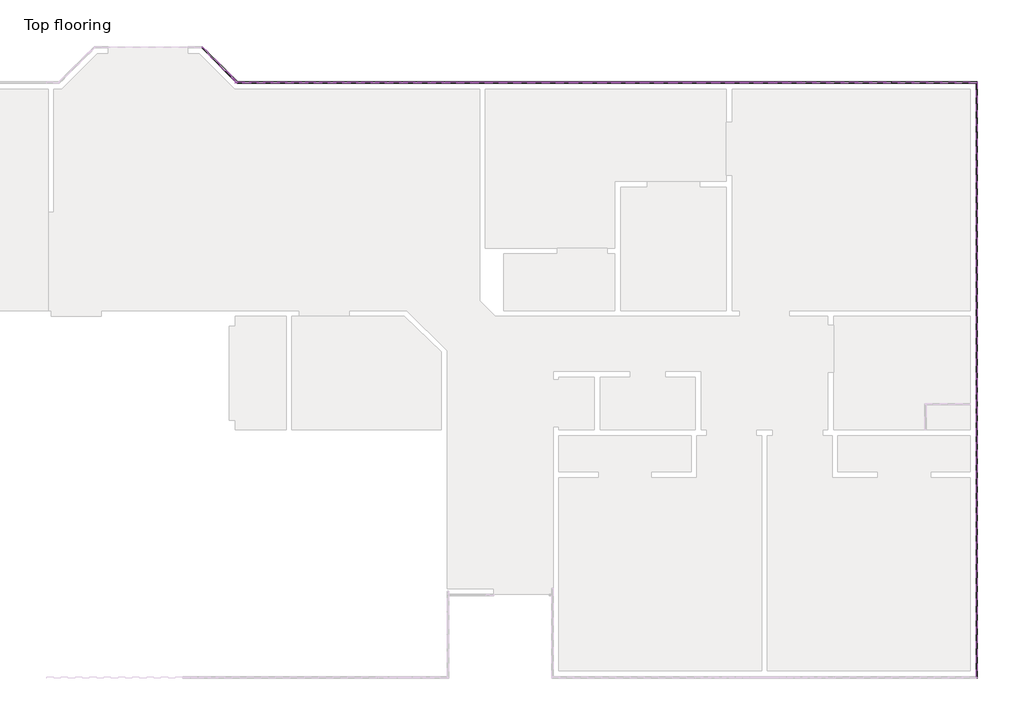
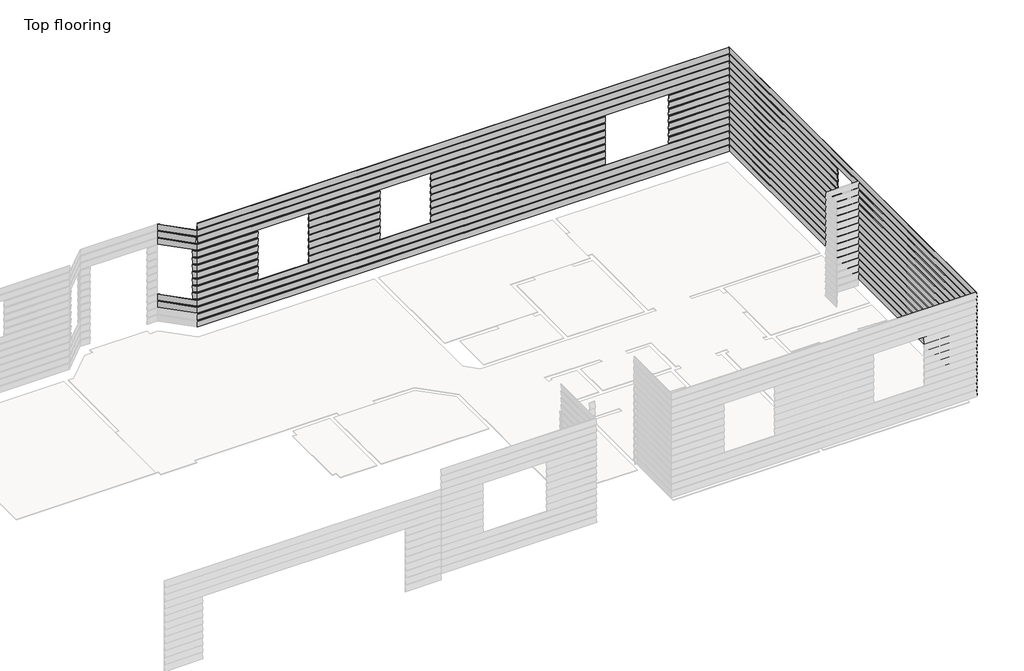
# One storey, part 5 of 5: 42 proxies.
"""IFC4 building model written with IfcOpenShell, lengths in millimetres."""

from ifc_helpers import new_model, si_unit, origin, place, context, project, spatial, faceted_brep, element, save

model = new_model("IFC4")

# Units and contexts
model_context = context("Model", 3, world=origin())
ifc_project = project(units=[si_unit("LENGTHUNIT", "METRE", prefix="MILLI")], contexts=[model_context])

# Site, building, storey
site = spatial("IfcSite", under=ifc_project)
building = spatial("IfcBuilding", under=site)
storey = spatial("IfcBuildingStorey", under=building, Name="Top flooring", Elevation=12.7)

# Proxies
placement = place(None, origin())
element("IfcBuildingElementProxy", 1, Name="Wall Sweeps", at=placement, inside=storey, context=model_context, shape_type="Brep", body=[
    faceted_brep([(-11064.5752841, 5231.8645018, 534.9151454), (-11070.4469329, 5217.6890875, 694.2859634), (-11074.5727801, 5207.7284114, 693.4), (-11068.7011312, 5221.9038257, 534.029182), (-11674.1752841, 5841.4645018, 534.9151454), (-11678.3011312, 5831.5038257, 534.029182), (-11684.1727801, 5817.3284114, 693.4), (-11680.0469329, 5827.2890875, 694.2859634)], [[[0, 1, 2, 3]], [[4, 5, 6, 7]], [[1, 0, 4, 7]], [[2, 1, 7, 6]], [[3, 2, 6, 5]], [[0, 3, 5, 4]]]),
])
element("IfcBuildingElementProxy", 2, Name="Wall Sweeps", at=placement, inside=storey, context=model_context, shape_type="Brep", body=[
    faceted_brep([(-11064.5752841, 5231.8645018, 712.7151454), (-11070.4469329, 5217.6890875, 872.0859634), (-11074.5727801, 5207.7284114, 871.2), (-11068.7011312, 5221.9038257, 711.829182), (-11674.1752841, 5841.4645018, 712.7151454), (-11678.3011312, 5831.5038257, 711.829182), (-11684.1727801, 5817.3284114, 871.2), (-11680.0469329, 5827.2890875, 872.0859634)], [[[0, 1, 2, 3]], [[4, 5, 6, 7]], [[1, 0, 4, 7]], [[2, 1, 7, 6]], [[3, 2, 6, 5]], [[0, 3, 5, 4]]]),
])
element("IfcBuildingElementProxy", 3, Name="Wall Sweeps", at=placement, inside=storey, context=model_context, shape_type="Brep", body=[
    faceted_brep([(-11064.5752841, 5231.8645018, 890.5151454), (-11070.4469329, 5217.6890875, 1049.8859634), (-11074.5727801, 5207.7284114, 1049.0), (-11068.7011312, 5221.9038257, 889.629182), (-11135.1593781, 5302.4485958, 890.5151454), (-11142.2026397, 5295.4053342, 889.629182), (-11152.2261713, 5285.3818026, 1049.0), (-11145.1829097, 5292.4250642, 1049.8859634)], [[[0, 1, 2, 3]], [[4, 5, 6, 7]], [[1, 0, 4, 7]], [[2, 1, 7, 6]], [[3, 2, 6, 5]], [[0, 3, 5, 4]]]),
])
element("IfcBuildingElementProxy", 4, Name="Wall Sweeps", at=placement, inside=storey, context=model_context, shape_type="Brep", body=[
    faceted_brep([(-11064.5752841, 5231.8645018, 1068.3151454), (-11070.4469329, 5217.6890875, 1227.6859634), (-11074.5727801, 5207.7284114, 1226.8), (-11068.7011312, 5221.9038257, 1067.429182), (-11135.1593781, 5302.4485958, 1068.3151454), (-11142.2026397, 5295.4053342, 1067.429182), (-11152.2261713, 5285.3818026, 1226.8), (-11145.1829097, 5292.4250642, 1227.6859634)], [[[0, 1, 2, 3]], [[4, 5, 6, 7]], [[1, 0, 4, 7]], [[2, 1, 7, 6]], [[3, 2, 6, 5]], [[0, 3, 5, 4]]]),
])
element("IfcBuildingElementProxy", 5, Name="Wall Sweeps", at=placement, inside=storey, context=model_context, shape_type="Brep", body=[
    faceted_brep([(-11064.5752841, 5231.8645018, 1246.1151454), (-11070.4469329, 5217.6890875, 1405.4859634), (-11074.5727801, 5207.7284114, 1404.6), (-11068.7011312, 5221.9038257, 1245.229182), (-11135.1593781, 5302.4485958, 1246.1151454), (-11142.2026397, 5295.4053342, 1245.229182), (-11152.2261713, 5285.3818026, 1404.6), (-11145.1829097, 5292.4250642, 1405.4859634)], [[[0, 1, 2, 3]], [[4, 5, 6, 7]], [[1, 0, 4, 7]], [[2, 1, 7, 6]], [[3, 2, 6, 5]], [[0, 3, 5, 4]]]),
])
element("IfcBuildingElementProxy", 6, Name="Wall Sweeps", at=placement, inside=storey, context=model_context, shape_type="Brep", body=[
    faceted_brep([(-11064.5752841, 5231.8645018, 1423.9151454), (-11070.4469329, 5217.6890875, 1583.2859634), (-11074.5727801, 5207.7284114, 1582.4), (-11068.7011312, 5221.9038257, 1423.029182), (-11135.1593781, 5302.4485958, 1423.9151454), (-11142.2026397, 5295.4053342, 1423.029182), (-11152.2261713, 5285.3818026, 1582.4), (-11145.1829097, 5292.4250642, 1583.2859634)], [[[0, 1, 2, 3]], [[4, 5, 6, 7]], [[1, 0, 4, 7]], [[2, 1, 7, 6]], [[3, 2, 6, 5]], [[0, 3, 5, 4]]]),
])
element("IfcBuildingElementProxy", 7, Name="Wall Sweeps", at=placement, inside=storey, context=model_context, shape_type="Brep", body=[
    faceted_brep([(-11064.5752841, 5231.8645018, 1601.7151454), (-11070.4469329, 5217.6890875, 1761.0859634), (-11074.5727801, 5207.7284114, 1760.2), (-11068.7011312, 5221.9038257, 1600.829182), (-11135.1593781, 5302.4485958, 1601.7151454), (-11142.2026397, 5295.4053342, 1600.829182), (-11152.2261713, 5285.3818026, 1760.2), (-11145.1829097, 5292.4250642, 1761.0859634)], [[[0, 1, 2, 3]], [[4, 5, 6, 7]], [[1, 0, 4, 7]], [[2, 1, 7, 6]], [[3, 2, 6, 5]], [[0, 3, 5, 4]]]),
])
element("IfcBuildingElementProxy", 8, Name="Wall Sweeps", at=placement, inside=storey, context=model_context, shape_type="Brep", body=[
    faceted_brep([(-11064.5752841, 5231.8645018, 1779.5151454), (-11070.4469329, 5217.6890875, 1938.8859634), (-11074.5727801, 5207.7284114, 1938.0), (-11068.7011312, 5221.9038257, 1778.629182), (-11135.1593781, 5302.4485958, 1779.5151454), (-11142.2026397, 5295.4053342, 1778.629182), (-11152.2261713, 5285.3818026, 1938.0), (-11145.1829097, 5292.4250642, 1938.8859634)], [[[0, 1, 2, 3]], [[4, 5, 6, 7]], [[1, 0, 4, 7]], [[2, 1, 7, 6]], [[3, 2, 6, 5]], [[0, 3, 5, 4]]]),
])
element("IfcBuildingElementProxy", 9, Name="Wall Sweeps", at=placement, inside=storey, context=model_context, shape_type="Brep", body=[
    faceted_brep([(-11064.5752841, 5231.8645018, 1957.3151454), (-11070.4469329, 5217.6890875, 2116.6859634), (-11074.5727801, 5207.7284114, 2115.8), (-11068.7011312, 5221.9038257, 1956.429182), (-11135.1593781, 5302.4485958, 1957.3151454), (-11142.2026397, 5295.4053342, 1956.429182), (-11152.2261713, 5285.3818026, 2115.8), (-11145.1829097, 5292.4250642, 2116.6859634)], [[[0, 1, 2, 3]], [[4, 5, 6, 7]], [[1, 0, 4, 7]], [[2, 1, 7, 6]], [[3, 2, 6, 5]], [[0, 3, 5, 4]]]),
])
element("IfcBuildingElementProxy", 10, Name="Wall Sweeps", at=placement, inside=storey, context=model_context, shape_type="Brep", body=[
    faceted_brep([(-11064.5752841, 5231.8645018, 2135.1151454), (-11070.4469329, 5217.6890875, 2294.4859634), (-11074.5727801, 5207.7284114, 2293.6), (-11068.7011312, 5221.9038257, 2134.229182), (-11674.1752841, 5841.4645018, 2135.1151454), (-11678.3011312, 5831.5038257, 2134.229182), (-11684.1727801, 5817.3284114, 2293.6), (-11680.0469329, 5827.2890875, 2294.4859634)], [[[0, 1, 2, 3]], [[4, 5, 6, 7]], [[1, 0, 4, 7]], [[2, 1, 7, 6]], [[3, 2, 6, 5]], [[0, 3, 5, 4]]]),
])
element("IfcBuildingElementProxy", 11, Name="Wall Sweeps", at=placement, inside=storey, context=model_context, shape_type="Brep", body=[
    faceted_brep([(1730.1212614, -5078.007679, 179.3151454), (1715.9458471, -5063.8322648, 338.6859634), (1705.985171, -5053.8715886, 337.8), (1720.1605853, -5068.0470029, 178.429182), (1730.1212614, 5231.8645018, 179.3151454), (1720.1605853, 5221.9038257, 178.429182), (1705.985171, 5207.7284114, 337.8), (1715.9458471, 5217.6890875, 338.6859634)], [[[0, 1, 2, 3]], [[4, 5, 6, 7]], [[1, 0, 4, 7]], [[2, 1, 7, 6]], [[3, 2, 6, 5]], [[0, 3, 5, 4]]]),
])
element("IfcBuildingElementProxy", 12, Name="Wall Sweeps", at=placement, inside=storey, context=model_context, shape_type="Brep", body=[
    faceted_brep([(1730.1212614, -5078.007679, 357.1151454), (1715.9458471, -5063.8322648, 516.4859634), (1705.985171, -5053.8715886, 515.6), (1720.1605853, -5068.0470029, 356.229182), (1730.1212614, 5231.8645018, 357.1151454), (1720.1605853, 5221.9038257, 356.229182), (1705.985171, 5207.7284114, 515.6), (1715.9458471, 5217.6890875, 516.4859634)], [[[0, 1, 2, 3]], [[4, 5, 6, 7]], [[1, 0, 4, 7]], [[2, 1, 7, 6]], [[3, 2, 6, 5]], [[0, 3, 5, 4]]]),
])
element("IfcBuildingElementProxy", 13, Name="Wall Sweeps", at=placement, inside=storey, context=model_context, shape_type="Brep", body=[
    faceted_brep([(1730.1212614, -5078.007679, 534.9151454), (1715.9458471, -5063.8322648, 694.2859634), (1705.985171, -5053.8715886, 693.4), (1720.1605853, -5068.0470029, 534.029182), (1730.1212614, 5231.8645018, 534.9151454), (1720.1605853, 5221.9038257, 534.029182), (1705.985171, 5207.7284114, 693.4), (1715.9458471, 5217.6890875, 694.2859634)], [[[0, 1, 2, 3]], [[4, 5, 6, 7]], [[1, 0, 4, 7]], [[2, 1, 7, 6]], [[3, 2, 6, 5]], [[0, 3, 5, 4]]]),
])
element("IfcBuildingElementProxy", 14, Name="Wall Sweeps", at=placement, inside=storey, context=model_context, shape_type="Brep", body=[
    faceted_brep([(1730.1212614, -5078.007679, 712.7151454), (1715.9458471, -5063.8322648, 872.0859634), (1705.985171, -5053.8715886, 871.2), (1720.1605853, -5068.0470029, 711.829182), (1730.1212614, 5231.8645018, 712.7151454), (1720.1605853, 5221.9038257, 711.829182), (1705.985171, 5207.7284114, 871.2), (1715.9458471, 5217.6890875, 872.0859634)], [[[0, 1, 2, 3]], [[4, 5, 6, 7]], [[1, 0, 4, 7]], [[2, 1, 7, 6]], [[3, 2, 6, 5]], [[0, 3, 5, 4]]]),
])
element("IfcBuildingElementProxy", 15, Name="Wall Sweeps", at=placement, inside=storey, context=model_context, shape_type="Brep", body=[
    faceted_brep([(1730.1212614, -5078.007679, 890.5151454), (1715.9458471, -5063.8322648, 1049.8859634), (1705.985171, -5053.8715886, 1049.0), (1720.1605853, -5068.0470029, 889.629182), (1730.1212614, 5231.8645018, 890.5151454), (1720.1605853, 5221.9038257, 889.629182), (1705.985171, 5207.7284114, 1049.0), (1715.9458471, 5217.6890875, 1049.8859634)], [[[0, 1, 2, 3]], [[4, 5, 6, 7]], [[1, 0, 4, 7]], [[2, 1, 7, 6]], [[3, 2, 6, 5]], [[0, 3, 5, 4]]]),
])
element("IfcBuildingElementProxy", 16, Name="Wall Sweeps", at=placement, inside=storey, context=model_context, shape_type="Brep", body=[
    faceted_brep([(1730.1212614, -5078.007679, 1068.3151454), (1715.9458471, -5063.8322648, 1227.6859634), (1705.985171, -5053.8715886, 1226.8), (1720.1605853, -5068.0470029, 1067.429182), (1730.1212614, 5231.8645018, 1068.3151454), (1720.1605853, 5221.9038257, 1067.429182), (1705.985171, 5207.7284114, 1226.8), (1715.9458471, 5217.6890875, 1227.6859634)], [[[0, 1, 2, 3]], [[4, 5, 6, 7]], [[1, 0, 4, 7]], [[2, 1, 7, 6]], [[3, 2, 6, 5]], [[0, 3, 5, 4]]]),
])
element("IfcBuildingElementProxy", 17, Name="Wall Sweeps", at=placement, inside=storey, context=model_context, shape_type="Brep", body=[
    faceted_brep([(1730.1212614, -5078.007679, 1246.1151454), (1715.9458471, -5063.8322648, 1405.4859634), (1705.985171, -5053.8715886, 1404.6), (1720.1605853, -5068.0470029, 1245.229182), (1730.1212614, 5231.8645018, 1246.1151454), (1720.1605853, 5221.9038257, 1245.229182), (1705.985171, 5207.7284114, 1404.6), (1715.9458471, 5217.6890875, 1405.4859634)], [[[0, 1, 2, 3]], [[4, 5, 6, 7]], [[1, 0, 4, 7]], [[2, 1, 7, 6]], [[3, 2, 6, 5]], [[0, 3, 5, 4]]]),
])
element("IfcBuildingElementProxy", 18, Name="Wall Sweeps", at=placement, inside=storey, context=model_context, shape_type="Brep", body=[
    faceted_brep([(1730.1212614, -5078.007679, 1423.9151454), (1715.9458471, -5063.8322648, 1583.2859634), (1705.985171, -5053.8715886, 1582.4), (1720.1605853, -5068.0470029, 1423.029182), (1730.1212614, 5231.8645018, 1423.9151454), (1720.1605853, 5221.9038257, 1423.029182), (1705.985171, 5207.7284114, 1582.4), (1715.9458471, 5217.6890875, 1583.2859634)], [[[0, 1, 2, 3]], [[4, 5, 6, 7]], [[1, 0, 4, 7]], [[2, 1, 7, 6]], [[3, 2, 6, 5]], [[0, 3, 5, 4]]]),
])
element("IfcBuildingElementProxy", 19, Name="Wall Sweeps", at=placement, inside=storey, context=model_context, shape_type="Brep", body=[
    faceted_brep([(1730.1212614, -5078.007679, 1601.7151454), (1715.9458471, -5063.8322648, 1761.0859634), (1705.985171, -5053.8715886, 1760.2), (1720.1605853, -5068.0470029, 1600.829182), (1730.1212614, 5231.8645018, 1601.7151454), (1720.1605853, 5221.9038257, 1600.829182), (1705.985171, 5207.7284114, 1760.2), (1715.9458471, 5217.6890875, 1761.0859634)], [[[0, 1, 2, 3]], [[4, 5, 6, 7]], [[1, 0, 4, 7]], [[2, 1, 7, 6]], [[3, 2, 6, 5]], [[0, 3, 5, 4]]]),
])
element("IfcBuildingElementProxy", 20, Name="Wall Sweeps", at=placement, inside=storey, context=model_context, shape_type="Brep", body=[
    faceted_brep([(1730.1212614, -5078.007679, 1779.5151454), (1715.9458471, -5063.8322648, 1938.8859634), (1705.985171, -5053.8715886, 1938.0), (1720.1605853, -5068.0470029, 1778.629182), (1730.1212614, 5231.8645018, 1779.5151454), (1720.1605853, 5221.9038257, 1778.629182), (1705.985171, 5207.7284114, 1938.0), (1715.9458471, 5217.6890875, 1938.8859634)], [[[0, 1, 2, 3]], [[4, 5, 6, 7]], [[1, 0, 4, 7]], [[2, 1, 7, 6]], [[3, 2, 6, 5]], [[0, 3, 5, 4]]]),
])
element("IfcBuildingElementProxy", 21, Name="Wall Sweeps", at=placement, inside=storey, context=model_context, shape_type="Brep", body=[
    faceted_brep([(1730.1212614, -5078.007679, 1957.3151454), (1715.9458471, -5063.8322648, 2116.6859634), (1705.985171, -5053.8715886, 2115.8), (1720.1605853, -5068.0470029, 1956.429182), (1730.1212614, 102.3284114, 1957.3151454), (1720.1605853, 102.3284114, 1956.429182), (1705.985171, 102.3284114, 2115.8), (1715.9458471, 102.3284114, 2116.6859634)], [[[0, 1, 2, 3]], [[4, 5, 6, 7]], [[1, 0, 4, 7]], [[2, 1, 7, 6]], [[3, 2, 6, 5]], [[0, 3, 5, 4]]]),
    faceted_brep([(1730.1212614, 711.9284114, 1957.3151454), (1715.9458471, 711.9284114, 2116.6859634), (1705.985171, 711.9284114, 2115.8), (1720.1605853, 711.9284114, 1956.429182), (1730.1212614, 5231.8645018, 1957.3151454), (1720.1605853, 5221.9038257, 1956.429182), (1705.985171, 5207.7284114, 2115.8), (1715.9458471, 5217.6890875, 2116.6859634)], [[[0, 1, 2, 3]], [[4, 5, 6, 7]], [[1, 0, 4, 7]], [[2, 1, 7, 6]], [[3, 2, 6, 5]], [[0, 3, 5, 4]]]),
])
element("IfcBuildingElementProxy", 22, Name="Wall Sweeps", at=placement, inside=storey, context=model_context, shape_type="Brep", body=[
    faceted_brep([(1730.1212614, -5078.007679, 2135.1151454), (1715.9458471, -5063.8322648, 2294.4859634), (1705.985171, -5053.8715886, 2293.6), (1720.1605853, -5068.0470029, 2134.229182), (1730.1212614, 102.3284114, 2135.1151454), (1720.1605853, 102.3284114, 2134.229182), (1705.985171, 102.3284114, 2293.6), (1715.9458471, 102.3284114, 2294.4859634)], [[[0, 1, 2, 3]], [[4, 5, 6, 7]], [[1, 0, 4, 7]], [[2, 1, 7, 6]], [[3, 2, 6, 5]], [[0, 3, 5, 4]]]),
    faceted_brep([(1730.1212614, 711.9284114, 2135.1151454), (1715.9458471, 711.9284114, 2294.4859634), (1705.985171, 711.9284114, 2293.6), (1720.1605853, 711.9284114, 2134.229182), (1730.1212614, 5231.8645018, 2135.1151454), (1720.1605853, 5221.9038257, 2134.229182), (1705.985171, 5207.7284114, 2293.6), (1715.9458471, 5217.6890875, 2294.4859634)], [[[0, 1, 2, 3]], [[4, 5, 6, 7]], [[1, 0, 4, 7]], [[2, 1, 7, 6]], [[3, 2, 6, 5]], [[0, 3, 5, 4]]]),
])
element("IfcBuildingElementProxy", 23, Name="Wall Sweeps", at=placement, inside=storey, context=model_context, shape_type="Brep", body=[
    faceted_brep([(1730.1212614, 5231.8645018, 179.3151454), (1715.9458471, 5217.6890875, 338.6859634), (1705.985171, 5207.7284114, 337.8), (1720.1605853, 5221.9038257, 178.429182), (-11064.5752841, 5231.8645018, 179.3151454), (-11068.7011312, 5221.9038257, 178.429182), (-11074.5727801, 5207.7284114, 337.8), (-11070.4469329, 5217.6890875, 338.6859634)], [[[0, 1, 2, 3]], [[4, 5, 6, 7]], [[1, 0, 4, 7]], [[2, 1, 7, 6]], [[3, 2, 6, 5]], [[0, 3, 5, 4]]]),
])
element("IfcBuildingElementProxy", 24, Name="Wall Sweeps", at=placement, inside=storey, context=model_context, shape_type="Brep", body=[
    faceted_brep([(1730.1212614, 5231.8645018, 357.1151454), (1715.9458471, 5217.6890875, 516.4859634), (1705.985171, 5207.7284114, 515.6), (1720.1605853, 5221.9038257, 356.229182), (-11064.5752841, 5231.8645018, 357.1151454), (-11068.7011312, 5221.9038257, 356.229182), (-11074.5727801, 5207.7284114, 515.6), (-11070.4469329, 5217.6890875, 516.4859634)], [[[0, 1, 2, 3]], [[4, 5, 6, 7]], [[1, 0, 4, 7]], [[2, 1, 7, 6]], [[3, 2, 6, 5]], [[0, 3, 5, 4]]]),
])
element("IfcBuildingElementProxy", 25, Name="Wall Sweeps", at=placement, inside=storey, context=model_context, shape_type="Brep", body=[
    faceted_brep([(1730.1212614, 5231.8645018, 534.9151454), (1715.9458471, 5217.6890875, 694.2859634), (1705.985171, 5207.7284114, 693.4), (1720.1605853, 5221.9038257, 534.029182), (-11064.5752841, 5231.8645018, 534.9151454), (-11068.7011312, 5221.9038257, 534.029182), (-11074.5727801, 5207.7284114, 693.4), (-11070.4469329, 5217.6890875, 694.2859634)], [[[0, 1, 2, 3]], [[4, 5, 6, 7]], [[1, 0, 4, 7]], [[2, 1, 7, 6]], [[3, 2, 6, 5]], [[0, 3, 5, 4]]]),
])
element("IfcBuildingElementProxy", 26, Name="Wall Sweeps", at=placement, inside=storey, context=model_context, shape_type="Brep", body=[
    faceted_brep([(1730.1212614, 5231.8645018, 712.7151454), (1715.9458471, 5217.6890875, 872.0859634), (1705.985171, 5207.7284114, 871.2), (1720.1605853, 5221.9038257, 711.829182), (-11064.5752841, 5231.8645018, 712.7151454), (-11068.7011312, 5221.9038257, 711.829182), (-11074.5727801, 5207.7284114, 871.2), (-11070.4469329, 5217.6890875, 872.0859634)], [[[0, 1, 2, 3]], [[4, 5, 6, 7]], [[1, 0, 4, 7]], [[2, 1, 7, 6]], [[3, 2, 6, 5]], [[0, 3, 5, 4]]]),
])
element("IfcBuildingElementProxy", 27, Name="Wall Sweeps", at=placement, inside=storey, context=model_context, shape_type="Brep", body=[
    faceted_brep([(1730.1212614, 5231.8645018, 890.5151454), (1715.9458471, 5217.6890875, 1049.8859634), (1705.985171, 5207.7284114, 1049.0), (1720.1605853, 5221.9038257, 889.629182), (251.835171, 5231.8645018, 890.5151454), (251.835171, 5221.9038257, 889.629182), (251.835171, 5207.7284114, 1049.0), (251.835171, 5217.6890875, 1049.8859634)], [[[0, 1, 2, 3]], [[4, 5, 6, 7]], [[1, 0, 4, 7]], [[2, 1, 7, 6]], [[3, 2, 6, 5]], [[0, 3, 5, 4]]]),
    faceted_brep([(-1272.164829, 5231.8645018, 890.5151454), (-1272.164829, 5217.6890875, 1049.8859634), (-1272.164829, 5207.7284114, 1049.0), (-1272.164829, 5221.9038257, 889.629182), (-5463.164829, 5231.8645018, 890.5151454), (-5463.164829, 5221.9038257, 889.629182), (-5463.164829, 5207.7284114, 1049.0), (-5463.164829, 5217.6890875, 1049.8859634)], [[[0, 1, 2, 3]], [[4, 5, 6, 7]], [[1, 0, 4, 7]], [[2, 1, 7, 6]], [[3, 2, 6, 5]], [[0, 3, 5, 4]]]),
    faceted_brep([(-6682.364829, 5231.8645018, 890.5151454), (-6682.364829, 5217.6890875, 1049.8859634), (-6682.364829, 5207.7284114, 1049.0), (-6682.364829, 5221.9038257, 889.629182), (-8396.864829, 5231.8645018, 890.5151454), (-8396.864829, 5221.9038257, 889.629182), (-8396.864829, 5207.7284114, 1049.0), (-8396.864829, 5217.6890875, 1049.8859634)], [[[0, 1, 2, 3]], [[4, 5, 6, 7]], [[1, 0, 4, 7]], [[2, 1, 7, 6]], [[3, 2, 6, 5]], [[0, 3, 5, 4]]]),
    faceted_brep([(-9616.064829, 5231.8645018, 890.5151454), (-9616.064829, 5217.6890875, 1049.8859634), (-9616.064829, 5207.7284114, 1049.0), (-9616.064829, 5221.9038257, 889.629182), (-11064.5752841, 5231.8645018, 890.5151454), (-11068.7011312, 5221.9038257, 889.629182), (-11074.5727801, 5207.7284114, 1049.0), (-11070.4469329, 5217.6890875, 1049.8859634)], [[[0, 1, 2, 3]], [[4, 5, 6, 7]], [[1, 0, 4, 7]], [[2, 1, 7, 6]], [[3, 2, 6, 5]], [[0, 3, 5, 4]]]),
])
element("IfcBuildingElementProxy", 28, Name="Wall Sweeps", at=placement, inside=storey, context=model_context, shape_type="Brep", body=[
    faceted_brep([(-9616.064829, 5231.8645018, 1068.3151454), (-9616.064829, 5217.6890875, 1227.6859634), (-9616.064829, 5207.7284114, 1226.8), (-9616.064829, 5221.9038257, 1067.429182), (-11064.5752841, 5231.8645018, 1068.3151454), (-11068.7011312, 5221.9038257, 1067.429182), (-11074.5727801, 5207.7284114, 1226.8), (-11070.4469329, 5217.6890875, 1227.6859634)], [[[0, 1, 2, 3]], [[4, 5, 6, 7]], [[1, 0, 4, 7]], [[2, 1, 7, 6]], [[3, 2, 6, 5]], [[0, 3, 5, 4]]]),
    faceted_brep([(-6682.364829, 5231.8645018, 1068.3151454), (-6682.364829, 5217.6890875, 1227.6859634), (-6682.364829, 5207.7284114, 1226.8), (-6682.364829, 5221.9038257, 1067.429182), (-8396.864829, 5231.8645018, 1068.3151454), (-8396.864829, 5221.9038257, 1067.429182), (-8396.864829, 5207.7284114, 1226.8), (-8396.864829, 5217.6890875, 1227.6859634)], [[[0, 1, 2, 3]], [[4, 5, 6, 7]], [[1, 0, 4, 7]], [[2, 1, 7, 6]], [[3, 2, 6, 5]], [[0, 3, 5, 4]]]),
    faceted_brep([(-1272.164829, 5231.8645018, 1068.3151454), (-1272.164829, 5217.6890875, 1227.6859634), (-1272.164829, 5207.7284114, 1226.8), (-1272.164829, 5221.9038257, 1067.429182), (-5463.164829, 5231.8645018, 1068.3151454), (-5463.164829, 5221.9038257, 1067.429182), (-5463.164829, 5207.7284114, 1226.8), (-5463.164829, 5217.6890875, 1227.6859634)], [[[0, 1, 2, 3]], [[4, 5, 6, 7]], [[1, 0, 4, 7]], [[2, 1, 7, 6]], [[3, 2, 6, 5]], [[0, 3, 5, 4]]]),
    faceted_brep([(1730.1212614, 5231.8645018, 1068.3151454), (1715.9458471, 5217.6890875, 1227.6859634), (1705.985171, 5207.7284114, 1226.8), (1720.1605853, 5221.9038257, 1067.429182), (251.835171, 5231.8645018, 1068.3151454), (251.835171, 5221.9038257, 1067.429182), (251.835171, 5207.7284114, 1226.8), (251.835171, 5217.6890875, 1227.6859634)], [[[0, 1, 2, 3]], [[4, 5, 6, 7]], [[1, 0, 4, 7]], [[2, 1, 7, 6]], [[3, 2, 6, 5]], [[0, 3, 5, 4]]]),
])
element("IfcBuildingElementProxy", 29, Name="Wall Sweeps", at=placement, inside=storey, context=model_context, shape_type="Brep", body=[
    faceted_brep([(-9616.064829, 5231.8645018, 1246.1151454), (-9616.064829, 5217.6890875, 1405.4859634), (-9616.064829, 5207.7284114, 1404.6), (-9616.064829, 5221.9038257, 1245.229182), (-11064.5752841, 5231.8645018, 1246.1151454), (-11068.7011312, 5221.9038257, 1245.229182), (-11074.5727801, 5207.7284114, 1404.6), (-11070.4469329, 5217.6890875, 1405.4859634)], [[[0, 1, 2, 3]], [[4, 5, 6, 7]], [[1, 0, 4, 7]], [[2, 1, 7, 6]], [[3, 2, 6, 5]], [[0, 3, 5, 4]]]),
    faceted_brep([(-6682.364829, 5231.8645018, 1246.1151454), (-6682.364829, 5217.6890875, 1405.4859634), (-6682.364829, 5207.7284114, 1404.6), (-6682.364829, 5221.9038257, 1245.229182), (-8396.864829, 5231.8645018, 1246.1151454), (-8396.864829, 5221.9038257, 1245.229182), (-8396.864829, 5207.7284114, 1404.6), (-8396.864829, 5217.6890875, 1405.4859634)], [[[0, 1, 2, 3]], [[4, 5, 6, 7]], [[1, 0, 4, 7]], [[2, 1, 7, 6]], [[3, 2, 6, 5]], [[0, 3, 5, 4]]]),
    faceted_brep([(-1272.164829, 5231.8645018, 1246.1151454), (-1272.164829, 5217.6890875, 1405.4859634), (-1272.164829, 5207.7284114, 1404.6), (-1272.164829, 5221.9038257, 1245.229182), (-5463.164829, 5231.8645018, 1246.1151454), (-5463.164829, 5221.9038257, 1245.229182), (-5463.164829, 5207.7284114, 1404.6), (-5463.164829, 5217.6890875, 1405.4859634)], [[[0, 1, 2, 3]], [[4, 5, 6, 7]], [[1, 0, 4, 7]], [[2, 1, 7, 6]], [[3, 2, 6, 5]], [[0, 3, 5, 4]]]),
    faceted_brep([(1730.1212614, 5231.8645018, 1246.1151454), (1715.9458471, 5217.6890875, 1405.4859634), (1705.985171, 5207.7284114, 1404.6), (1720.1605853, 5221.9038257, 1245.229182), (251.835171, 5231.8645018, 1246.1151454), (251.835171, 5221.9038257, 1245.229182), (251.835171, 5207.7284114, 1404.6), (251.835171, 5217.6890875, 1405.4859634)], [[[0, 1, 2, 3]], [[4, 5, 6, 7]], [[1, 0, 4, 7]], [[2, 1, 7, 6]], [[3, 2, 6, 5]], [[0, 3, 5, 4]]]),
])
element("IfcBuildingElementProxy", 30, Name="Wall Sweeps", at=placement, inside=storey, context=model_context, shape_type="Brep", body=[
    faceted_brep([(-9616.064829, 5231.8645018, 1423.9151454), (-9616.064829, 5217.6890875, 1583.2859634), (-9616.064829, 5207.7284114, 1582.4), (-9616.064829, 5221.9038257, 1423.029182), (-11064.5752841, 5231.8645018, 1423.9151454), (-11068.7011312, 5221.9038257, 1423.029182), (-11074.5727801, 5207.7284114, 1582.4), (-11070.4469329, 5217.6890875, 1583.2859634)], [[[0, 1, 2, 3]], [[4, 5, 6, 7]], [[1, 0, 4, 7]], [[2, 1, 7, 6]], [[3, 2, 6, 5]], [[0, 3, 5, 4]]]),
    faceted_brep([(-6682.364829, 5231.8645018, 1423.9151454), (-6682.364829, 5217.6890875, 1583.2859634), (-6682.364829, 5207.7284114, 1582.4), (-6682.364829, 5221.9038257, 1423.029182), (-8396.864829, 5231.8645018, 1423.9151454), (-8396.864829, 5221.9038257, 1423.029182), (-8396.864829, 5207.7284114, 1582.4), (-8396.864829, 5217.6890875, 1583.2859634)], [[[0, 1, 2, 3]], [[4, 5, 6, 7]], [[1, 0, 4, 7]], [[2, 1, 7, 6]], [[3, 2, 6, 5]], [[0, 3, 5, 4]]]),
    faceted_brep([(-1272.164829, 5231.8645018, 1423.9151454), (-1272.164829, 5217.6890875, 1583.2859634), (-1272.164829, 5207.7284114, 1582.4), (-1272.164829, 5221.9038257, 1423.029182), (-5463.164829, 5231.8645018, 1423.9151454), (-5463.164829, 5221.9038257, 1423.029182), (-5463.164829, 5207.7284114, 1582.4), (-5463.164829, 5217.6890875, 1583.2859634)], [[[0, 1, 2, 3]], [[4, 5, 6, 7]], [[1, 0, 4, 7]], [[2, 1, 7, 6]], [[3, 2, 6, 5]], [[0, 3, 5, 4]]]),
    faceted_brep([(1730.1212614, 5231.8645018, 1423.9151454), (1715.9458471, 5217.6890875, 1583.2859634), (1705.985171, 5207.7284114, 1582.4), (1720.1605853, 5221.9038257, 1423.029182), (251.835171, 5231.8645018, 1423.9151454), (251.835171, 5221.9038257, 1423.029182), (251.835171, 5207.7284114, 1582.4), (251.835171, 5217.6890875, 1583.2859634)], [[[0, 1, 2, 3]], [[4, 5, 6, 7]], [[1, 0, 4, 7]], [[2, 1, 7, 6]], [[3, 2, 6, 5]], [[0, 3, 5, 4]]]),
])
element("IfcBuildingElementProxy", 31, Name="Wall Sweeps", at=placement, inside=storey, context=model_context, shape_type="Brep", body=[
    faceted_brep([(-9616.064829, 5231.8645018, 1601.7151454), (-9616.064829, 5217.6890875, 1761.0859634), (-9616.064829, 5207.7284114, 1760.2), (-9616.064829, 5221.9038257, 1600.829182), (-11064.5752841, 5231.8645018, 1601.7151454), (-11068.7011312, 5221.9038257, 1600.829182), (-11074.5727801, 5207.7284114, 1760.2), (-11070.4469329, 5217.6890875, 1761.0859634)], [[[0, 1, 2, 3]], [[4, 5, 6, 7]], [[1, 0, 4, 7]], [[2, 1, 7, 6]], [[3, 2, 6, 5]], [[0, 3, 5, 4]]]),
    faceted_brep([(-6682.364829, 5231.8645018, 1601.7151454), (-6682.364829, 5217.6890875, 1761.0859634), (-6682.364829, 5207.7284114, 1760.2), (-6682.364829, 5221.9038257, 1600.829182), (-8396.864829, 5231.8645018, 1601.7151454), (-8396.864829, 5221.9038257, 1600.829182), (-8396.864829, 5207.7284114, 1760.2), (-8396.864829, 5217.6890875, 1761.0859634)], [[[0, 1, 2, 3]], [[4, 5, 6, 7]], [[1, 0, 4, 7]], [[2, 1, 7, 6]], [[3, 2, 6, 5]], [[0, 3, 5, 4]]]),
    faceted_brep([(-1272.164829, 5231.8645018, 1601.7151454), (-1272.164829, 5217.6890875, 1761.0859634), (-1272.164829, 5207.7284114, 1760.2), (-1272.164829, 5221.9038257, 1600.829182), (-5463.164829, 5231.8645018, 1601.7151454), (-5463.164829, 5221.9038257, 1600.829182), (-5463.164829, 5207.7284114, 1760.2), (-5463.164829, 5217.6890875, 1761.0859634)], [[[0, 1, 2, 3]], [[4, 5, 6, 7]], [[1, 0, 4, 7]], [[2, 1, 7, 6]], [[3, 2, 6, 5]], [[0, 3, 5, 4]]]),
    faceted_brep([(1730.1212614, 5231.8645018, 1601.7151454), (1715.9458471, 5217.6890875, 1761.0859634), (1705.985171, 5207.7284114, 1760.2), (1720.1605853, 5221.9038257, 1600.829182), (251.835171, 5231.8645018, 1601.7151454), (251.835171, 5221.9038257, 1600.829182), (251.835171, 5207.7284114, 1760.2), (251.835171, 5217.6890875, 1761.0859634)], [[[0, 1, 2, 3]], [[4, 5, 6, 7]], [[1, 0, 4, 7]], [[2, 1, 7, 6]], [[3, 2, 6, 5]], [[0, 3, 5, 4]]]),
])
element("IfcBuildingElementProxy", 32, Name="Wall Sweeps", at=placement, inside=storey, context=model_context, shape_type="Brep", body=[
    faceted_brep([(-9616.064829, 5231.8645018, 1779.5151454), (-9616.064829, 5217.6890875, 1938.8859634), (-9616.064829, 5207.7284114, 1938.0), (-9616.064829, 5221.9038257, 1778.629182), (-11064.5752841, 5231.8645018, 1779.5151454), (-11068.7011312, 5221.9038257, 1778.629182), (-11074.5727801, 5207.7284114, 1938.0), (-11070.4469329, 5217.6890875, 1938.8859634)], [[[0, 1, 2, 3]], [[4, 5, 6, 7]], [[1, 0, 4, 7]], [[2, 1, 7, 6]], [[3, 2, 6, 5]], [[0, 3, 5, 4]]]),
    faceted_brep([(-6682.364829, 5231.8645018, 1779.5151454), (-6682.364829, 5217.6890875, 1938.8859634), (-6682.364829, 5207.7284114, 1938.0), (-6682.364829, 5221.9038257, 1778.629182), (-8396.864829, 5231.8645018, 1779.5151454), (-8396.864829, 5221.9038257, 1778.629182), (-8396.864829, 5207.7284114, 1938.0), (-8396.864829, 5217.6890875, 1938.8859634)], [[[0, 1, 2, 3]], [[4, 5, 6, 7]], [[1, 0, 4, 7]], [[2, 1, 7, 6]], [[3, 2, 6, 5]], [[0, 3, 5, 4]]]),
    faceted_brep([(-1272.164829, 5231.8645018, 1779.5151454), (-1272.164829, 5217.6890875, 1938.8859634), (-1272.164829, 5207.7284114, 1938.0), (-1272.164829, 5221.9038257, 1778.629182), (-5463.164829, 5231.8645018, 1779.5151454), (-5463.164829, 5221.9038257, 1778.629182), (-5463.164829, 5207.7284114, 1938.0), (-5463.164829, 5217.6890875, 1938.8859634)], [[[0, 1, 2, 3]], [[4, 5, 6, 7]], [[1, 0, 4, 7]], [[2, 1, 7, 6]], [[3, 2, 6, 5]], [[0, 3, 5, 4]]]),
    faceted_brep([(1730.1212614, 5231.8645018, 1779.5151454), (1715.9458471, 5217.6890875, 1938.8859634), (1705.985171, 5207.7284114, 1938.0), (1720.1605853, 5221.9038257, 1778.629182), (251.835171, 5231.8645018, 1779.5151454), (251.835171, 5221.9038257, 1778.629182), (251.835171, 5207.7284114, 1938.0), (251.835171, 5217.6890875, 1938.8859634)], [[[0, 1, 2, 3]], [[4, 5, 6, 7]], [[1, 0, 4, 7]], [[2, 1, 7, 6]], [[3, 2, 6, 5]], [[0, 3, 5, 4]]]),
])
element("IfcBuildingElementProxy", 33, Name="Wall Sweeps", at=placement, inside=storey, context=model_context, shape_type="Brep", body=[
    faceted_brep([(-9616.064829, 5231.8645018, 1957.3151454), (-9616.064829, 5217.6890875, 2116.6859634), (-9616.064829, 5207.7284114, 2115.8), (-9616.064829, 5221.9038257, 1956.429182), (-11064.5752841, 5231.8645018, 1957.3151454), (-11068.7011312, 5221.9038257, 1956.429182), (-11074.5727801, 5207.7284114, 2115.8), (-11070.4469329, 5217.6890875, 2116.6859634)], [[[0, 1, 2, 3]], [[4, 5, 6, 7]], [[1, 0, 4, 7]], [[2, 1, 7, 6]], [[3, 2, 6, 5]], [[0, 3, 5, 4]]]),
    faceted_brep([(-6682.364829, 5231.8645018, 1957.3151454), (-6682.364829, 5217.6890875, 2116.6859634), (-6682.364829, 5207.7284114, 2115.8), (-6682.364829, 5221.9038257, 1956.429182), (-8396.864829, 5231.8645018, 1957.3151454), (-8396.864829, 5221.9038257, 1956.429182), (-8396.864829, 5207.7284114, 2115.8), (-8396.864829, 5217.6890875, 2116.6859634)], [[[0, 1, 2, 3]], [[4, 5, 6, 7]], [[1, 0, 4, 7]], [[2, 1, 7, 6]], [[3, 2, 6, 5]], [[0, 3, 5, 4]]]),
    faceted_brep([(-1272.164829, 5231.8645018, 1957.3151454), (-1272.164829, 5217.6890875, 2116.6859634), (-1272.164829, 5207.7284114, 2115.8), (-1272.164829, 5221.9038257, 1956.429182), (-5463.164829, 5231.8645018, 1957.3151454), (-5463.164829, 5221.9038257, 1956.429182), (-5463.164829, 5207.7284114, 2115.8), (-5463.164829, 5217.6890875, 2116.6859634)], [[[0, 1, 2, 3]], [[4, 5, 6, 7]], [[1, 0, 4, 7]], [[2, 1, 7, 6]], [[3, 2, 6, 5]], [[0, 3, 5, 4]]]),
    faceted_brep([(1730.1212614, 5231.8645018, 1957.3151454), (1715.9458471, 5217.6890875, 2116.6859634), (1705.985171, 5207.7284114, 2115.8), (1720.1605853, 5221.9038257, 1956.429182), (251.835171, 5231.8645018, 1957.3151454), (251.835171, 5221.9038257, 1956.429182), (251.835171, 5207.7284114, 2115.8), (251.835171, 5217.6890875, 2116.6859634)], [[[0, 1, 2, 3]], [[4, 5, 6, 7]], [[1, 0, 4, 7]], [[2, 1, 7, 6]], [[3, 2, 6, 5]], [[0, 3, 5, 4]]]),
])
element("IfcBuildingElementProxy", 34, Name="Wall Sweeps", at=placement, inside=storey, context=model_context, shape_type="Brep", body=[
    faceted_brep([(1730.1212614, 5231.8645018, 2135.1151454), (1715.9458471, 5217.6890875, 2294.4859634), (1705.985171, 5207.7284114, 2293.6), (1720.1605853, 5221.9038257, 2134.229182), (-11064.5752841, 5231.8645018, 2135.1151454), (-11068.7011312, 5221.9038257, 2134.229182), (-11074.5727801, 5207.7284114, 2293.6), (-11070.4469329, 5217.6890875, 2294.4859634)], [[[0, 1, 2, 3]], [[4, 5, 6, 7]], [[1, 0, 4, 7]], [[2, 1, 7, 6]], [[3, 2, 6, 5]], [[0, 3, 5, 4]]]),
])
element("IfcBuildingElementProxy", 35, Name="Wall Sweeps", at=placement, inside=storey, context=model_context, shape_type="Brep", body=[
    faceted_brep([(-11057.5059869, 5224.7952046, 2312.9151454), (-11067.5295184, 5214.771673, 2472.2859634), (-11074.5727801, 5207.7284114, 2471.4), (-11064.5492485, 5217.7519429, 2312.029182), (-11674.1752841, 5841.4645018, 2312.9151454), (-11678.3011312, 5831.5038257, 2312.029182), (-11684.1727801, 5817.3284114, 2471.4), (-11680.0469329, 5827.2890875, 2472.2859634)], [[[0, 1, 2, 3]], [[4, 5, 6, 7]], [[1, 0, 4, 7]], [[2, 1, 7, 6]], [[3, 2, 6, 5]], [[0, 3, 5, 4]]]),
])
element("IfcBuildingElementProxy", 36, Name="Wall Sweeps", at=placement, inside=storey, context=model_context, shape_type="Brep", body=[
    faceted_brep([(-11064.5752841, 5231.8645018, 2490.7151454), (-11070.4469329, 5217.6890875, 2650.0859634), (-11074.5727801, 5207.7284114, 2649.2), (-11068.7011312, 5221.9038257, 2489.829182), (-11674.1752841, 5841.4645018, 2490.7151454), (-11678.3011312, 5831.5038257, 2489.829182), (-11684.1727801, 5817.3284114, 2649.2), (-11680.0469329, 5827.2890875, 2650.0859634)], [[[0, 1, 2, 3]], [[4, 5, 6, 7]], [[1, 0, 4, 7]], [[2, 1, 7, 6]], [[3, 2, 6, 5]], [[0, 3, 5, 4]]]),
])
element("IfcBuildingElementProxy", 37, Name="Wall Sweeps", at=placement, inside=storey, context=model_context, shape_type="Brep", body=[
    faceted_brep([(1730.1212614, 711.9284114, 2312.9151454), (1715.9458471, 711.9284114, 2472.2859634), (1705.985171, 711.9284114, 2471.4), (1720.1605853, 711.9284114, 2312.029182), (1730.1212614, 5231.8645018, 2312.9151454), (1720.1605853, 5221.9038257, 2312.029182), (1705.985171, 5207.7284114, 2471.4), (1715.9458471, 5217.6890875, 2472.2859634)], [[[0, 1, 2, 3]], [[4, 5, 6, 7]], [[1, 0, 4, 7]], [[2, 1, 7, 6]], [[3, 2, 6, 5]], [[0, 3, 5, 4]]]),
    faceted_brep([(1730.1212614, -5078.007679, 2312.9151454), (1715.9458471, -5063.8322648, 2472.2859634), (1705.985171, -5053.8715886, 2471.4), (1720.1605853, -5068.0470029, 2312.029182), (1730.1212614, 102.3284114, 2312.9151454), (1720.1605853, 102.3284114, 2312.029182), (1705.985171, 102.3284114, 2471.4), (1715.9458471, 102.3284114, 2472.2859634)], [[[0, 1, 2, 3]], [[4, 5, 6, 7]], [[1, 0, 4, 7]], [[2, 1, 7, 6]], [[3, 2, 6, 5]], [[0, 3, 5, 4]]]),
])
element("IfcBuildingElementProxy", 38, Name="Wall Sweeps", at=placement, inside=storey, context=model_context, shape_type="Brep", body=[
    faceted_brep([(1730.1212614, -5078.007679, 2490.7151454), (1715.9458471, -5063.8322648, 2650.0859634), (1705.985171, -5053.8715886, 2649.2), (1720.1605853, -5068.0470029, 2489.829182), (1730.1212614, 5231.8645018, 2490.7151454), (1720.1605853, 5221.9038257, 2489.829182), (1705.985171, 5207.7284114, 2649.2), (1715.9458471, 5217.6890875, 2650.0859634)], [[[0, 1, 2, 3]], [[4, 5, 6, 7]], [[1, 0, 4, 7]], [[2, 1, 7, 6]], [[3, 2, 6, 5]], [[0, 3, 5, 4]]]),
])
element("IfcBuildingElementProxy", 39, Name="Wall Sweeps", at=placement, inside=storey, context=model_context, shape_type="Brep", body=[
    faceted_brep([(1730.1212614, 5231.8645018, 2312.9151454), (1715.9458471, 5217.6890875, 2472.2859634), (1705.985171, 5207.7284114, 2471.4), (1720.1605853, 5221.9038257, 2312.029182), (-11101.964829, 5231.8645018, 2312.9151454), (-11101.964829, 5221.9038257, 2312.029182), (-11101.964829, 5207.7284114, 2471.4), (-11101.964829, 5217.6890875, 2472.2859634)], [[[0, 1, 2, 3]], [[4, 5, 6, 7]], [[1, 0, 4, 7]], [[2, 1, 7, 6]], [[3, 2, 6, 5]], [[0, 3, 5, 4]]]),
])
element("IfcBuildingElementProxy", 40, Name="Wall Sweeps", at=placement, inside=storey, context=model_context, shape_type="Brep", body=[
    faceted_brep([(1730.1212614, 5231.8645018, 2490.7151454), (1715.9458471, 5217.6890875, 2650.0859634), (1705.985171, 5207.7284114, 2649.2), (1720.1605853, 5221.9038257, 2489.829182), (-11064.5752841, 5231.8645018, 2490.7151454), (-11068.7011312, 5221.9038257, 2489.829182), (-11074.5727801, 5207.7284114, 2649.2), (-11070.4469329, 5217.6890875, 2650.0859634)], [[[0, 1, 2, 3]], [[4, 5, 6, 7]], [[1, 0, 4, 7]], [[2, 1, 7, 6]], [[3, 2, 6, 5]], [[0, 3, 5, 4]]]),
])
element("IfcBuildingElementProxy", 41, Name="Wall Sweeps", at=placement, inside=storey, context=model_context, shape_type="Brep", body=[
    faceted_brep([(1730.1212614, -5078.007679, 2668.5151454), (1715.9458471, -5063.8322648, 2827.8859634), (1705.985171, -5053.8715886, 2827.0), (1720.1605853, -5068.0470029, 2667.629182), (1730.1212614, 5231.8645018, 2668.5151454), (1720.1605853, 5221.9038257, 2667.629182), (1705.985171, 5207.7284114, 2827.0), (1715.9458471, 5217.6890875, 2827.8859634)], [[[0, 1, 2, 3]], [[4, 5, 6, 7]], [[1, 0, 4, 7]], [[2, 1, 7, 6]], [[3, 2, 6, 5]], [[0, 3, 5, 4]]]),
])
element("IfcBuildingElementProxy", 42, Name="Wall Sweeps", at=placement, inside=storey, context=model_context, shape_type="Brep", body=[
    faceted_brep([(1730.1212614, 5231.8645018, 2668.5151454), (1715.9458471, 5217.6890875, 2827.8859634), (1705.985171, 5207.7284114, 2827.0), (1720.1605853, 5221.9038257, 2667.629182), (-11074.5727801, 5231.8645018, 2668.5151454), (-11074.5727801, 5221.9038257, 2667.629182), (-11074.5727801, 5207.7284114, 2827.0), (-11074.5727801, 5217.6890875, 2827.8859634)], [[[0, 1, 2, 3]], [[4, 5, 6, 7]], [[1, 0, 4, 7]], [[2, 1, 7, 6]], [[3, 2, 6, 5]], [[0, 3, 5, 4]]]),
])

save(model, "model.ifc")

# Revit data of these elements
# Elements 1, 2, 3, 4, 5, 6, 7, 8, 9, 10, 11, 12, 13, 14, 15, 16, 17, 18, 19, 20, 21, 22, 23, 24, 25, 26, 27, 28, 29, 30, 31, 32, 33, 34, 35, 36, 37, 38, 39, 40, 41, 42 (IfcBuildingElementProxy)
#   Phase Created = New Construction
#   Materials on its faces: "Aluminum"
# Materials
#   "Aluminum": class "Metal", colour RGB 244 244 244, transparency 0, Description = "Aluminum 6061", Cost = 0
